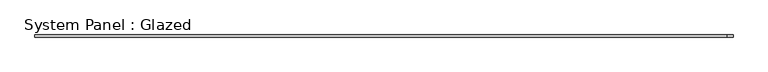
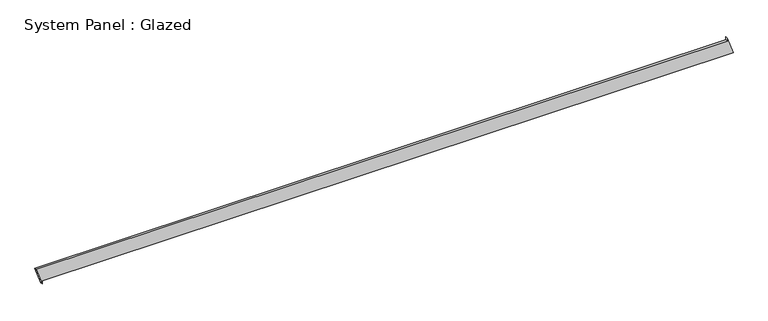
"""IFC4 building model written with IfcOpenShell, lengths in millimetres: plate geometry, System Panel : Glazed."""

from ifc_helpers import new_model, si_unit, frame, origin, place, context, project, spatial, polyline, outline, extrude, source, transform, mapped, element, save


def system_panel_glazed_efea60a0(model_context):
    return source(origin(), model_context, "Body", "SweptSolid", [
        extrude(outline(polyline([(0.0, -3959.0814895), (35.3553391, -3959.0814895), (35.3553391, 4028.0476561), (235.7077234, 3959.2529397), (200.3523843, 3959.2532528), (200.2816694, -4028.0476561), (0.0, -3959.0814895)])), frame((0.0, -49.5, 0.0), z_axis=(0.0, 1.0, 0.0), x_axis=(0.0, 0.0, 1.0)), (0.0, 0.0, 1.0), 25.0),
    ])


if __name__ == "__main__":
    model = new_model("IFC4")
    model_context = context("Model", 3, world=origin())
    ifc_project = project(units=[si_unit("LENGTHUNIT", "METRE", prefix="MILLI")], contexts=[model_context])
    site = spatial("IfcSite", under=ifc_project)
    building = spatial("IfcBuilding", under=site)
    placement = place(None, origin())
    system_panel_glazed_shape = system_panel_glazed_efea60a0(model_context)
    element("IfcPlate", 1, ObjectType="System Panel : Glazed", at=placement, inside=building, context=model_context, shape_type="MappedRepresentation", body=[
        mapped(system_panel_glazed_shape, transform((0.0, 0.0, 0.0), x_axis=(1.0, 0.0, 0.0), y_axis=(0.0, 1.0, 0.0), z_axis=(0.0, 0.0, 1.0))),
    ])
    save(model, "model.ifc")

# Revit data of these elements
# Element 1 (IfcPlate, "System Panel : Glazed")
#   Materials on its faces: "Glass"
# Materials
#   "Glass": class "Glass", colour RGB 218 227 224, transparency 0.85, Description = "Soda Lime Glass", Cost = 0
